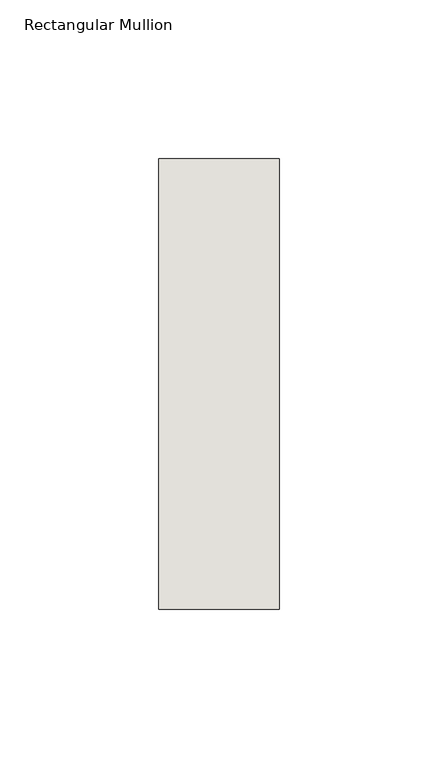
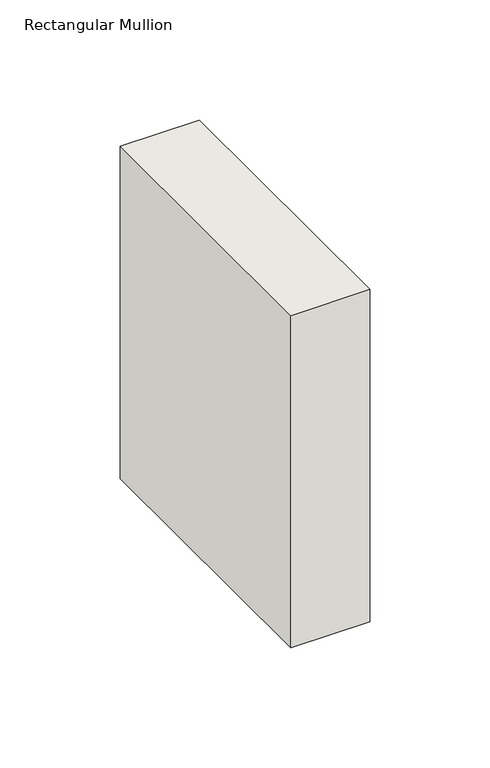
"""IFC4 building model written with IfcOpenShell, lengths in millimetres: wall geometry, Rectangular Mullion : NLRS_21_CWM_hsb-regel 38x142_gen_rsf."""

import ifcopenshell
import ifcopenshell.guid

model = None  # the IFC model being written
_history = None  # IfcOwnerHistory: only IFC2X3 demands one
_inside = {}  # id of a spatial element -> (the spatial element, [elements in it])
_under = {}  # id of a project, library or spatial element -> (it, [spatial elements below it])
_declared = {}  # id of a project -> (the project, [libraries it declares])
_typed = {}  # id of a type object -> (the type object, [elements of that type])
_made_of = {}  # id of a material, layer set ... -> (it, [elements and type objects made of it])


def new_model(schema):
    """Start an empty IFC model of exactly this schema.

    Asked for "IFC4X3", IfcOpenShell would pick the latest addendum, in which some entities
    have other attributes; the version numbers below select the first issue.
    IFC2X3 requires an IfcOwnerHistory on every rooted entity: one is made here for all.
    """
    global model, _history
    if schema == "IFC4X3":
        model = ifcopenshell.file(schema_version=(4, 3, 0, 0))
    else:
        model = ifcopenshell.file(schema=schema)
    _inside.clear()
    _under.clear()
    _declared.clear()
    _typed.clear()
    _made_of.clear()
    _history = None
    if model.schema == "IFC2X3":
        org = make("IfcOrganization", Name="unknown")
        user = make(
            "IfcPersonAndOrganization",
            ThePerson=make("IfcPerson", FamilyName="unknown"),
            TheOrganization=org,
        )
        app = make(
            "IfcApplication",
            ApplicationDeveloper=org,
            Version="unknown",
            ApplicationFullName="unknown",
            ApplicationIdentifier="unknown",
        )
        _history = make(
            "IfcOwnerHistory",
            OwningUser=user,
            OwningApplication=app,
            ChangeAction="ADDED",
            CreationDate=0,
        )
    return model


def make(cls, **values):
    """One entity of the class cls with the attributes given. An attribute that is None is left unset."""
    return model.create_entity(
        cls, **{name: value for name, value in values.items() if value is not None}
    )


def rooted(cls, **values):
    """An entity with a GlobalId (a new one), such as an element, a storey or a relation."""
    return make(cls, GlobalId=ifcopenshell.guid.new(), OwnerHistory=_history, **values)


def si_unit(unit_type, name, prefix=None):
    """IfcSIUnit, for example si_unit("LENGTHUNIT", "METRE", prefix="MILLI")."""
    return make("IfcSIUnit", UnitType=unit_type, Prefix=prefix, Name=name)


def assignment(units):
    """IfcUnitAssignment: the units of a project."""
    return None if units is None else make("IfcUnitAssignment", Units=units)


def point(xyz):
    """IfcCartesianPoint."""
    return None if xyz is None else make("IfcCartesianPoint", Coordinates=xyz)


def direction(xyz):
    """IfcDirection."""
    return None if xyz is None else make("IfcDirection", DirectionRatios=xyz)


def frame(location, z_axis=None, x_axis=None):
    """IfcAxis2Placement3D, a coordinate frame: its origin and axes. An axis left out is left unset."""
    return make(
        "IfcAxis2Placement3D",
        Location=point(location),
        Axis=direction(z_axis),
        RefDirection=direction(x_axis),
    )


def origin():
    """The frame at (0, 0, 0) with its axes left unset."""
    return frame((0.0, 0.0, 0.0))


def place(relative_to, where):
    """IfcLocalPlacement: puts the frame where relative to a parent placement (None: the world)."""
    return make(
        "IfcLocalPlacement", PlacementRelTo=relative_to, RelativePlacement=where
    )


def context(
    kind, dimensions, precision=None, world=None, true_north=None, identifier=None
):
    """IfcGeometricRepresentationContext, for example the 3D "Model" context."""
    return make(
        "IfcGeometricRepresentationContext",
        ContextIdentifier=identifier,
        ContextType=kind,
        CoordinateSpaceDimension=dimensions,
        Precision=precision,
        WorldCoordinateSystem=world,
        TrueNorth=true_north,
    )


def project(units=None, contexts=None):
    """IfcProject with its units and contexts."""
    return rooted(
        "IfcProject",
        Name="project",
        RepresentationContexts=contexts,
        UnitsInContext=assignment(units),
    )


def spatial(cls, under=None, at=None, **own):
    """A site, building, storey or space (cls), placed at a placement, below another one or the project."""
    s = rooted(cls, ObjectPlacement=at, **own)
    if under is not None:
        _under.setdefault(under.id(), (under, []))[1].append(s)
    return s


def polyline(points):
    """IfcPolyline through the points."""
    return make("IfcPolyline", Points=[point(p) for p in points])


def outline(outer, holes=None, kind="AREA"):
    """IfcArbitraryClosedProfileDef: a profile drawn as a closed curve; with holes, ...WithVoids."""
    if holes is None:
        return make("IfcArbitraryClosedProfileDef", ProfileType=kind, OuterCurve=outer)
    return make(
        "IfcArbitraryProfileDefWithVoids",
        ProfileType=kind,
        OuterCurve=outer,
        InnerCurves=holes,
    )


def extrude(swept, where, along, depth):
    """IfcExtrudedAreaSolid: the profile swept, set in the frame where, extruded along a direction by depth."""
    return make(
        "IfcExtrudedAreaSolid",
        SweptArea=swept,
        Position=where,
        ExtrudedDirection=direction(along),
        Depth=depth,
    )


def shape(context_of_items, identifier, shape_type, items):
    """IfcShapeRepresentation: the items that make up one representation, for example the "Body"."""
    return make(
        "IfcShapeRepresentation",
        ContextOfItems=context_of_items,
        RepresentationIdentifier=identifier,
        RepresentationType=shape_type,
        Items=items,
    )


def source(mapping_origin, context_of_items, identifier, shape_type, items):
    """IfcRepresentationMap: a shape defined once, which mapped items show again and again."""
    return make(
        "IfcRepresentationMap",
        MappingOrigin=mapping_origin,
        MappedRepresentation=shape(context_of_items, identifier, shape_type, items),
    )


def transform(
    local_origin,
    x_axis=None,
    y_axis=None,
    z_axis=None,
    scale=None,
    scale2=None,
    scale3=None,
    uniform=True,
):
    """IfcCartesianTransformationOperator3D, or its non-uniform kind. x_axis, y_axis, z_axis: its Axis1, 2, 3."""
    if uniform:
        return make(
            "IfcCartesianTransformationOperator3D",
            Axis1=direction(x_axis),
            Axis2=direction(y_axis),
            LocalOrigin=point(local_origin),
            Scale=scale,
            Axis3=direction(z_axis),
        )
    return make(
        "IfcCartesianTransformationOperator3DnonUniform",
        Axis1=direction(x_axis),
        Axis2=direction(y_axis),
        LocalOrigin=point(local_origin),
        Scale=scale,
        Axis3=direction(z_axis),
        Scale2=scale2,
        Scale3=scale3,
    )


def mapped(mapping_source, mapping_target):
    """IfcMappedItem: shows the shape of a source again, moved by a transform."""
    return make(
        "IfcMappedItem", MappingSource=mapping_source, MappingTarget=mapping_target
    )


def made_of(thing, what):
    """Note that an element or type object is made of a material, layer set ...; save() writes the relation."""
    if what is not None:
        _made_of.setdefault(what.id(), (what, []))[1].append(thing)
    return thing


def element(
    cls,
    number,
    at=None,
    inside=None,
    cuts=None,
    type_object=None,
    material=None,
    context=None,
    identifier="Body",
    shape_type=None,
    held_by="IfcProductDefinitionShape",
    body=None,
    shapes=None,
    **own,
):
    """One element of the class cls, such as IfcWall. Its Tag is "e" and its number.

    at: its placement. inside: the storey or other place that contains it. cuts: it is an
    opening in that element (IfcRelVoidsElement). A single representation is given by context,
    identifier, shape_type and body (its items); several are given by shapes. held_by: the class
    of the entity that holds the representations. save() writes the other relations.
    """
    e = rooted(cls, Tag="e%d" % number, ObjectPlacement=at, **own)
    if body is not None:
        shapes = [shape(context, identifier, shape_type, body)]
    if shapes is not None:
        e.Representation = make(held_by, Representations=shapes)
    if inside is not None:
        _inside.setdefault(inside.id(), (inside, []))[1].append(e)
    if cuts is not None:
        rooted(
            "IfcRelVoidsElement", RelatingBuildingElement=cuts, RelatedOpeningElement=e
        )
    if type_object is not None:
        _typed.setdefault(type_object.id(), (type_object, []))[1].append(e)
    return made_of(e, material)


def aggregate(whole, parts):
    """IfcRelAggregates: a whole, such as a stair, and the parts it consists of."""
    return rooted("IfcRelAggregates", RelatingObject=whole, RelatedObjects=parts)


def save(model, path):
    """Write the relations noted so far, then the file.

    IfcRelAggregates (storeys below a building ...), IfcRelContainedInSpatialStructure (elements
    in a storey), IfcRelDefinesByType, IfcRelAssociatesMaterial and IfcRelDeclares: one each for
    every whole, place, type object, material and project.
    """
    for whole, parts in _under.values():
        aggregate(whole, parts)
    for where, things in _inside.values():
        rooted(
            "IfcRelContainedInSpatialStructure",
            RelatedElements=things,
            RelatingStructure=where,
        )
    for kind, things in _typed.values():
        rooted("IfcRelDefinesByType", RelatedObjects=things, RelatingType=kind)
    for what, things in _made_of.values():
        rooted("IfcRelAssociatesMaterial", RelatedObjects=things, RelatingMaterial=what)
    for by, libraries in _declared.values():
        rooted("IfcRelDeclares", RelatingContext=by, RelatedDefinitions=libraries)
    model.write(path)


def rectangular_mullion_fbae096f(model_context):
    return source(origin(), model_context, "Body", "SweptSolid", [
        extrude(outline(polyline([(-38.0, -71.0), (-38.0, 71.0), (0.0, 71.0), (0.0, -71.0), (-38.0, -71.0)])), frame((0.0, 0.0, -168.9999997), z_axis=(0.0, 0.0, 1.0), x_axis=(1.0, 0.0, 0.0)), (0.0, 0.0, 1.0), 168.9999997),
    ])


if __name__ == "__main__":
    model = new_model("IFC4")
    model_context = context("Model", 3, world=origin())
    ifc_project = project(units=[si_unit("LENGTHUNIT", "METRE", prefix="MILLI")], contexts=[model_context])
    site = spatial("IfcSite", under=ifc_project)
    building = spatial("IfcBuilding", under=site)
    placement = place(None, origin())
    rectangular_mullion_shape = rectangular_mullion_fbae096f(model_context)
    element("IfcWall", 1, ObjectType="Rectangular Mullion : NLRS_21_CWM_hsb-regel 38x142_gen_rsf", at=placement, inside=building, context=model_context, shape_type="MappedRepresentation", body=[
        mapped(rectangular_mullion_shape, transform((0.0, 0.0, 0.0), x_axis=(1.0, 0.0, 0.0), y_axis=(0.0, 1.0, 0.0), z_axis=(0.0, 0.0, 1.0))),
    ])
    save(model, "model.ifc")

# Revit data of these elements
# Type "Rectangular Mullion : NLRS_21_CWM_hsb-regel 38x142_gen_rsf"
#   Type IfcGUID = "07M7mRoiH1CR8m_RSKIwpF"
#   Assembly Code = "21.10"
#   IfcExportAs = "IfcWall"
#   built-in parameter 1007322 = 0.465879 (stored number, unit not read)
#   built-in parameter 1007321 = 0.062336 (stored number, unit not read)
#   built-in parameter 1007320 = 0.062336 (stored number, unit not read)
# Element 1 (IfcWall, "Rectangular Mullion : NLRS_21_CWM_hsb-regel 38x142_gen_rsf")
#   Materials on its faces: "NLRS_i2_hout naaldhout vuren_gen_rsf"
# Materials
#   "NLRS_i2_hout naaldhout vuren_gen_rsf": class "I - Hout", colour RGB 234 199 147, transparency 0, Keynote = "i2", Manufacturer = "Revit Standards Foundation", URL = "www.revitstandards.org", Description = "hout vuren", Cost = 0
